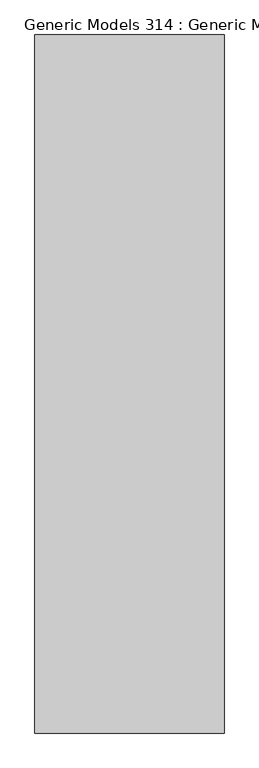
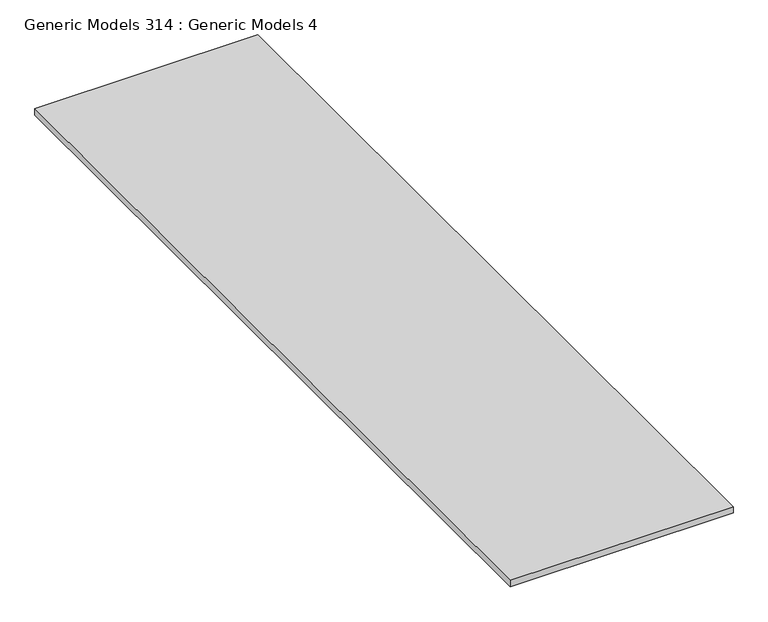
"""IFC4 building model written with IfcOpenShell, lengths in millimetres: proxy geometry, Generic Models 314 : Generic Models 4."""

from ifc_helpers import new_model, si_unit, frame, origin, place, context, project, spatial, polyline, outline, extrude, source, transform, mapped, element, save


def generic_models_314_generic_models_4_85dc28ef(model_context):
    return source(origin(), model_context, "Body", "SweptSolid", [
        extrude(outline(polyline([(-6629.5736296, -5493.3230338), (-10028.1472239, -5493.3230338), (-10028.1472239, 7054.2769662), (-6629.5736296, 7054.2769662), (-6629.5736296, -5493.3230338)])), frame((0.0, 0.0, 122803.2484874), z_axis=(0.0, 0.0, 1.0), x_axis=(1.0, 0.0, 0.0)), (0.0, 0.0, 1.0), 101.6),
    ])


if __name__ == "__main__":
    model = new_model("IFC4")
    model_context = context("Model", 3, world=origin())
    ifc_project = project(units=[si_unit("LENGTHUNIT", "METRE", prefix="MILLI")], contexts=[model_context])
    site = spatial("IfcSite", under=ifc_project)
    building = spatial("IfcBuilding", under=site)
    placement = place(None, origin())
    generic_models_314_generic_models_4_shape = generic_models_314_generic_models_4_85dc28ef(model_context)
    element("IfcBuildingElementProxy", 1, Name="Generic Models 314 : Generic Models 4", ObjectType="Generic Models 314 : Generic Models 4", at=placement, inside=building, context=model_context, shape_type="MappedRepresentation", body=[
        mapped(generic_models_314_generic_models_4_shape, transform((0.0, 0.0, 0.0), x_axis=(1.0, 0.0, 0.0), y_axis=(0.0, 1.0, 0.0), z_axis=(0.0, 0.0, 1.0))),
    ])
    save(model, "model.ifc")

# Revit data of these elements
# Element 1 (IfcBuildingElementProxy, "Generic Models 314 : Generic Models 4")
#   Materials on its faces: "_4\" MIN. CRUSHED GRAVEL (NO FINES)"
# Materials
#   "_4\" MIN. CRUSHED GRAVEL (NO FINES)": class "Generic", colour RGB 122 131 148, transparency 0, Cost = 0
